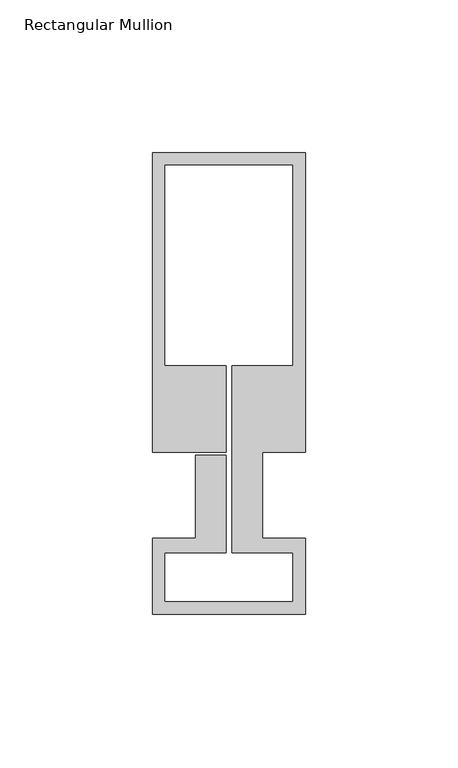
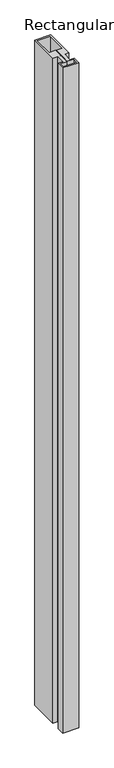
"""IFC4 building model written with IfcOpenShell, lengths in millimetres: member geometry, Rectangular Mullion : Schueco_FWS-50-HI_Mull_CovCap-20mm_Mull-85mm."""

from ifc_helpers import new_model, si_unit, frame, origin, place, context, project, spatial, polyline, outline, extrude, source, transform, mapped, element, save


def rectangular_mullion_14763fba(model_context):
    return source(origin(), model_context, "Body", "SweptSolid", [
        extrude(outline(polyline([(0.0, 126.0), (0.0, 28.0), (-14.0, 28.0), (-14.0, -0.1), (0.0, -0.1), (0.0, -25.0), (-50.0, -25.0), (-50.0, -0.1), (-36.0, -0.1), (-36.0, 27.0), (-26.0, 27.0), (-26.0, -5.0), (-46.0, -5.0), (-46.0, -21.0), (-4.0, -21.0), (-4.0, -5.0), (-24.0, -5.0), (-24.0, 56.3), (-4.0, 56.3), (-4.0, 122.0), (-46.0, 122.0), (-46.0, 56.3), (-26.0, 56.3), (-26.0, 28.0), (-50.0, 28.0), (-50.0, 126.0), (0.0, 126.0)])), frame((0.0, 0.0, -2200.0), z_axis=(0.0, 0.0, 1.0), x_axis=(1.0, 0.0, 0.0)), (0.0, 0.0, 1.0), 2200.0),
    ])


if __name__ == "__main__":
    model = new_model("IFC4")
    model_context = context("Model", 3, world=origin())
    ifc_project = project(units=[si_unit("LENGTHUNIT", "METRE", prefix="MILLI")], contexts=[model_context])
    site = spatial("IfcSite", under=ifc_project)
    building = spatial("IfcBuilding", under=site)
    placement = place(None, origin())
    rectangular_mullion_shape = rectangular_mullion_14763fba(model_context)
    element("IfcMember", 1, ObjectType="Rectangular Mullion : Schueco_FWS-50-HI_Mull_CovCap-20mm_Mull-85mm", at=placement, inside=building, context=model_context, shape_type="MappedRepresentation", body=[
        mapped(rectangular_mullion_shape, transform((0.0, 0.0, 0.0), x_axis=(1.0, 0.0, 0.0), y_axis=(0.0, 1.0, 0.0), z_axis=(0.0, 0.0, 1.0))),
    ])
    save(model, "model.ifc")

# Revit data of these elements
# Type "Rectangular Mullion : Schueco_FWS-50-HI_Mull_CovCap-20mm_Mull-85mm"
#   Model = "FWS 50.HI"
#   Manufacturer = "Schueco International KG"
#   Type Comments = "Mullion"
#   Schueco thermal insulation standard = "Highly thermally insulated"
#   Burglar resistance = "RC 3"
#   Thermal insulation = "to 0.90 W/(m²K)"
#   built-in parameter 1007322 = 0.495407 (stored number, unit not read)
#   built-in parameter 1007321 = 0.0360892 (stored number, unit not read)
#   built-in parameter 1007320 = 0.0360892 (stored number, unit not read)
# Element 1 (IfcMember, "Rectangular Mullion : Schueco_FWS-50-HI_Mull_CovCap-20mm_Mull-85mm")
#   Materials on its faces: "Alu"
# Materials
#   "Alu": class "Glas", colour RGB 140 140 140, transparency 0
